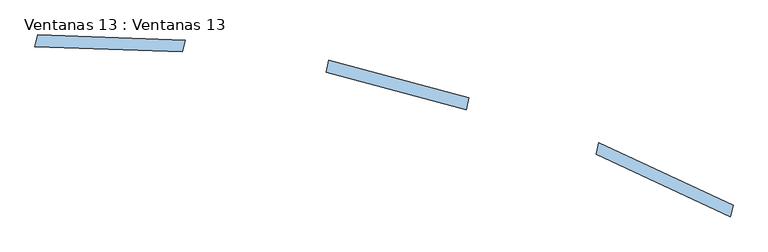
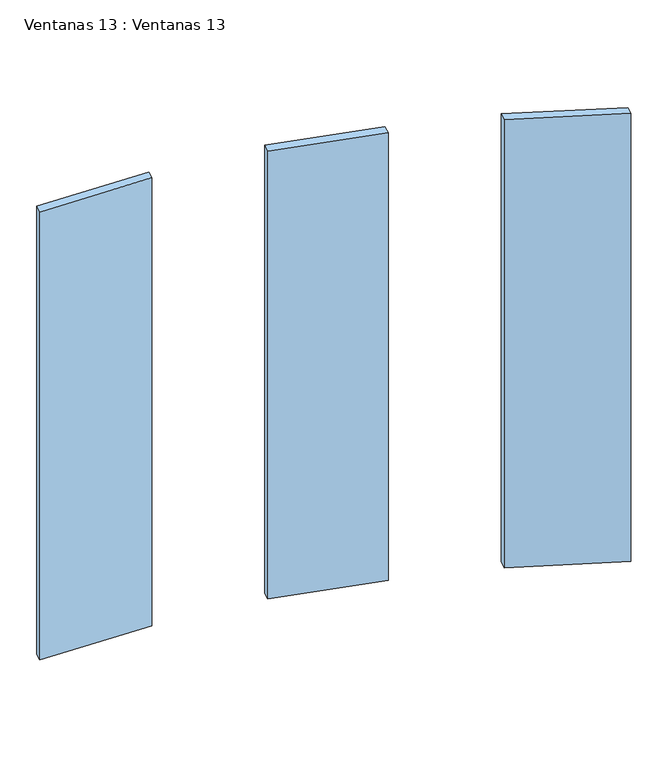
"""IFC4 building model written with IfcOpenShell, lengths in millimetres: window geometry, Ventanas 13 : Ventanas 13."""

from ifc_helpers import new_model, si_unit, frame, origin, place, context, project, spatial, polyline, outline, extrude, source, transform, mapped, element, save


def ventanas_13_ventanas_13_d0d4e7dc(model_context):
    return source(origin(), model_context, "Body", "SweptSolid", [
        extrude(outline(polyline([(-3391.5702432, 972.0182065), (-3396.0692643, 952.5308052), (-3640.4123331, 961.0634532), (-3635.913312, 980.5508545), (-3391.5702432, 972.0182065)])), frame((0.0, 0.0, 7117.1211204), z_axis=(0.0, 0.0, 1.0), x_axis=(1.0, 0.0, 0.0)), (0.0, 0.0, 1.0), 1055.5960323),
        extrude(outline(polyline([(-2921.0345633, 876.3346401), (-2925.5335844, 856.8472389), (-3157.4970886, 919.0016725), (-3152.9980675, 938.4890738), (-2921.0345633, 876.3346401)])), frame((0.0, 0.0, 7117.1211204), z_axis=(0.0, 0.0, 1.0), x_axis=(1.0, 0.0, 0.0)), (0.0, 0.0, 1.0), 1055.5960323),
        extrude(outline(polyline([(-2483.0170839, 698.3880269), (-2487.516105, 678.9006256), (-2709.8893631, 782.5949788), (-2705.390342, 802.0823801), (-2483.0170839, 698.3880269)])), frame((0.0, 0.0, 7117.1211204), z_axis=(0.0, 0.0, 1.0), x_axis=(1.0, 0.0, 0.0)), (0.0, 0.0, 1.0), 1055.5960323),
    ])


if __name__ == "__main__":
    model = new_model("IFC4")
    model_context = context("Model", 3, world=origin())
    ifc_project = project(units=[si_unit("LENGTHUNIT", "METRE", prefix="MILLI")], contexts=[model_context])
    site = spatial("IfcSite", under=ifc_project)
    building = spatial("IfcBuilding", under=site)
    placement = place(None, origin())
    ventanas_13_ventanas_13_shape = ventanas_13_ventanas_13_d0d4e7dc(model_context)
    element("IfcWindow", 1, ObjectType="Ventanas 13 : Ventanas 13", at=placement, inside=building, context=model_context, shape_type="MappedRepresentation", body=[
        mapped(ventanas_13_ventanas_13_shape, transform((0.0, 0.0, 0.0), x_axis=(1.0, 0.0, 0.0), y_axis=(0.0, 1.0, 0.0), z_axis=(0.0, 0.0, 1.0))),
    ])
    save(model, "model.ifc")

# Revit data of these elements
# Type "Ventanas 13 : Ventanas 13"
#   Type Mark = "39"
# Element 1 (IfcWindow, "Ventanas 13 : Ventanas 13")
#   Materials on its faces: "VIDRIO"
# Materials
#   "VIDRIO": class "Genérico", colour RGB 120 120 120, transparency 0, Cost = 0
